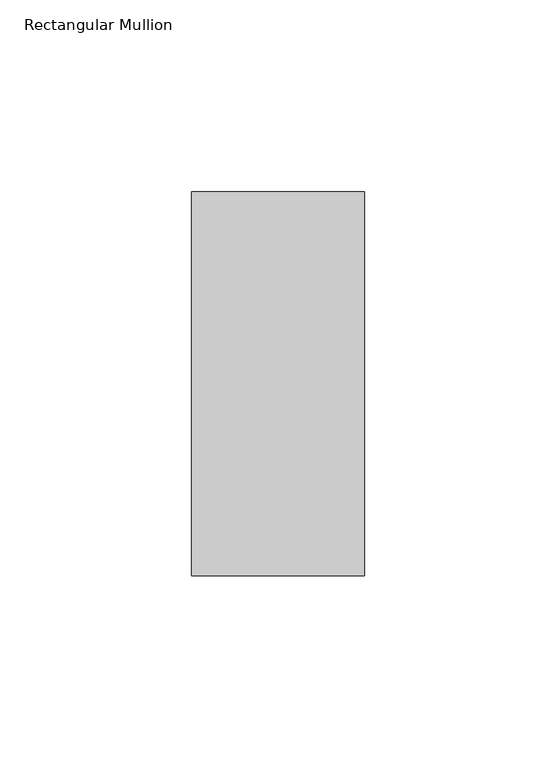
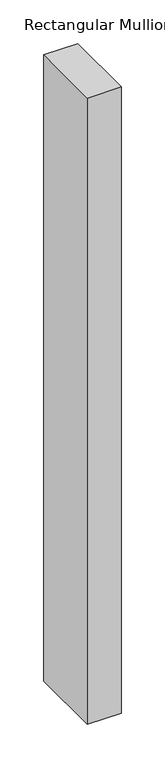
"""IFC4 building model written with IfcOpenShell, lengths in millimetres: member geometry, Rectangular Mullion : 알루미늄_Rectangular Cap_100 x 45."""

from ifc_helpers import new_model, si_unit, frame, origin, place, context, project, spatial, polyline, outline, extrude, source, transform, mapped, element, save


def rectangular_mullion_72d4057f(model_context):
    return source(origin(), model_context, "Body", "SweptSolid", [
        extrude(outline(polyline([(22.5, 50.0), (22.5, -50.0), (-22.5, -50.0), (-22.5, 50.0), (22.5, 50.0)])), frame((0.0, 0.0, -877.5), z_axis=(0.0, 0.0, 1.0), x_axis=(1.0, 0.0, 0.0)), (0.0, 0.0, 1.0), 877.5),
    ])


if __name__ == "__main__":
    model = new_model("IFC4")
    model_context = context("Model", 3, world=origin())
    ifc_project = project(units=[si_unit("LENGTHUNIT", "METRE", prefix="MILLI")], contexts=[model_context])
    site = spatial("IfcSite", under=ifc_project)
    building = spatial("IfcBuilding", under=site)
    placement = place(None, origin())
    rectangular_mullion_shape = rectangular_mullion_72d4057f(model_context)
    element("IfcMember", 1, ObjectType="Rectangular Mullion : 알루미늄_Rectangular Cap_100 x 45", at=placement, inside=building, context=model_context, shape_type="MappedRepresentation", body=[
        mapped(rectangular_mullion_shape, transform((0.0, 0.0, 0.0), x_axis=(1.0, 0.0, 0.0), y_axis=(0.0, 1.0, 0.0), z_axis=(0.0, 0.0, 1.0))),
    ])
    save(model, "model.ifc")

# Revit data of these elements
# Type "Rectangular Mullion : 알루미늄_Rectangular Cap_100 x 45"
#   built-in parameter 1007304 = 0.328084 (stored number, unit not read)
#   built-in parameter 1007301 = 0.0738189 (stored number, unit not read)
#   built-in parameter 1007300 = 0.0738189 (stored number, unit not read)
# Element 1 (IfcMember, "Rectangular Mullion : 알루미늄_Rectangular Cap_100 x 45")
#   Materials on its faces: "00_Metal_Stainless Steel"
# Materials
#   "00_Metal_Stainless Steel": class "Metal", colour RGB 148 148 148, transparency 0, Description = "Steel", Cost = 0
